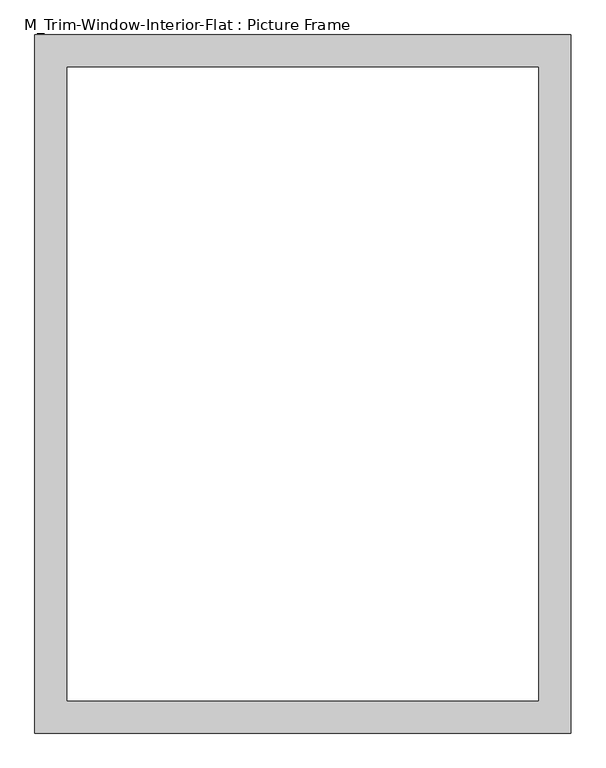
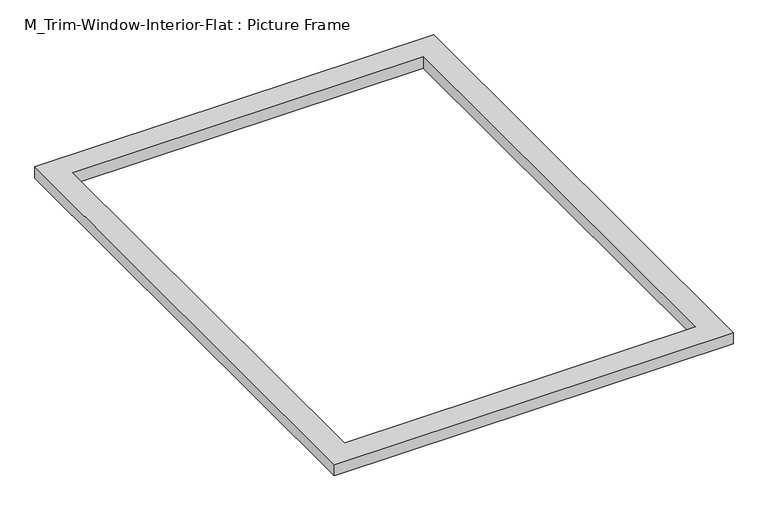
"""IFC4 building model written with IfcOpenShell, lengths in millimetres: proxy geometry, M_Trim-Window-Interior-Flat : Picture Frame."""

import ifcopenshell
import ifcopenshell.guid

model = None  # the IFC model being written
_history = None  # IfcOwnerHistory: only IFC2X3 demands one
_inside = {}  # id of a spatial element -> (the spatial element, [elements in it])
_under = {}  # id of a project, library or spatial element -> (it, [spatial elements below it])
_declared = {}  # id of a project -> (the project, [libraries it declares])
_typed = {}  # id of a type object -> (the type object, [elements of that type])
_made_of = {}  # id of a material, layer set ... -> (it, [elements and type objects made of it])


def new_model(schema):
    """Start an empty IFC model of exactly this schema.

    Asked for "IFC4X3", IfcOpenShell would pick the latest addendum, in which some entities
    have other attributes; the version numbers below select the first issue.
    IFC2X3 requires an IfcOwnerHistory on every rooted entity: one is made here for all.
    """
    global model, _history
    if schema == "IFC4X3":
        model = ifcopenshell.file(schema_version=(4, 3, 0, 0))
    else:
        model = ifcopenshell.file(schema=schema)
    _inside.clear()
    _under.clear()
    _declared.clear()
    _typed.clear()
    _made_of.clear()
    _history = None
    if model.schema == "IFC2X3":
        org = make("IfcOrganization", Name="unknown")
        user = make(
            "IfcPersonAndOrganization",
            ThePerson=make("IfcPerson", FamilyName="unknown"),
            TheOrganization=org,
        )
        app = make(
            "IfcApplication",
            ApplicationDeveloper=org,
            Version="unknown",
            ApplicationFullName="unknown",
            ApplicationIdentifier="unknown",
        )
        _history = make(
            "IfcOwnerHistory",
            OwningUser=user,
            OwningApplication=app,
            ChangeAction="ADDED",
            CreationDate=0,
        )
    return model


def make(cls, **values):
    """One entity of the class cls with the attributes given. An attribute that is None is left unset."""
    return model.create_entity(
        cls, **{name: value for name, value in values.items() if value is not None}
    )


def rooted(cls, **values):
    """An entity with a GlobalId (a new one), such as an element, a storey or a relation."""
    return make(cls, GlobalId=ifcopenshell.guid.new(), OwnerHistory=_history, **values)


def si_unit(unit_type, name, prefix=None):
    """IfcSIUnit, for example si_unit("LENGTHUNIT", "METRE", prefix="MILLI")."""
    return make("IfcSIUnit", UnitType=unit_type, Prefix=prefix, Name=name)


def assignment(units):
    """IfcUnitAssignment: the units of a project."""
    return None if units is None else make("IfcUnitAssignment", Units=units)


def point(xyz):
    """IfcCartesianPoint."""
    return None if xyz is None else make("IfcCartesianPoint", Coordinates=xyz)


def direction(xyz):
    """IfcDirection."""
    return None if xyz is None else make("IfcDirection", DirectionRatios=xyz)


def frame(location, z_axis=None, x_axis=None):
    """IfcAxis2Placement3D, a coordinate frame: its origin and axes. An axis left out is left unset."""
    return make(
        "IfcAxis2Placement3D",
        Location=point(location),
        Axis=direction(z_axis),
        RefDirection=direction(x_axis),
    )


def origin():
    """The frame at (0, 0, 0) with its axes left unset."""
    return frame((0.0, 0.0, 0.0))


def origin_with_axes():
    """The frame at (0, 0, 0) with the z axis (0, 0, 1) and the x axis (1, 0, 0) written out."""
    return frame((0.0, 0.0, 0.0), z_axis=(0.0, 0.0, 1.0), x_axis=(1.0, 0.0, 0.0))


def place(relative_to, where):
    """IfcLocalPlacement: puts the frame where relative to a parent placement (None: the world)."""
    return make(
        "IfcLocalPlacement", PlacementRelTo=relative_to, RelativePlacement=where
    )


def context(
    kind, dimensions, precision=None, world=None, true_north=None, identifier=None
):
    """IfcGeometricRepresentationContext, for example the 3D "Model" context."""
    return make(
        "IfcGeometricRepresentationContext",
        ContextIdentifier=identifier,
        ContextType=kind,
        CoordinateSpaceDimension=dimensions,
        Precision=precision,
        WorldCoordinateSystem=world,
        TrueNorth=true_north,
    )


def project(units=None, contexts=None):
    """IfcProject with its units and contexts."""
    return rooted(
        "IfcProject",
        Name="project",
        RepresentationContexts=contexts,
        UnitsInContext=assignment(units),
    )


def spatial(cls, under=None, at=None, **own):
    """A site, building, storey or space (cls), placed at a placement, below another one or the project."""
    s = rooted(cls, ObjectPlacement=at, **own)
    if under is not None:
        _under.setdefault(under.id(), (under, []))[1].append(s)
    return s


def polyline(points):
    """IfcPolyline through the points."""
    return make("IfcPolyline", Points=[point(p) for p in points])


def outline(outer, holes=None, kind="AREA"):
    """IfcArbitraryClosedProfileDef: a profile drawn as a closed curve; with holes, ...WithVoids."""
    if holes is None:
        return make("IfcArbitraryClosedProfileDef", ProfileType=kind, OuterCurve=outer)
    return make(
        "IfcArbitraryProfileDefWithVoids",
        ProfileType=kind,
        OuterCurve=outer,
        InnerCurves=holes,
    )


def extrude(swept, where, along, depth):
    """IfcExtrudedAreaSolid: the profile swept, set in the frame where, extruded along a direction by depth."""
    return make(
        "IfcExtrudedAreaSolid",
        SweptArea=swept,
        Position=where,
        ExtrudedDirection=direction(along),
        Depth=depth,
    )


def shape(context_of_items, identifier, shape_type, items):
    """IfcShapeRepresentation: the items that make up one representation, for example the "Body"."""
    return make(
        "IfcShapeRepresentation",
        ContextOfItems=context_of_items,
        RepresentationIdentifier=identifier,
        RepresentationType=shape_type,
        Items=items,
    )


def source(mapping_origin, context_of_items, identifier, shape_type, items):
    """IfcRepresentationMap: a shape defined once, which mapped items show again and again."""
    return make(
        "IfcRepresentationMap",
        MappingOrigin=mapping_origin,
        MappedRepresentation=shape(context_of_items, identifier, shape_type, items),
    )


def transform(
    local_origin,
    x_axis=None,
    y_axis=None,
    z_axis=None,
    scale=None,
    scale2=None,
    scale3=None,
    uniform=True,
):
    """IfcCartesianTransformationOperator3D, or its non-uniform kind. x_axis, y_axis, z_axis: its Axis1, 2, 3."""
    if uniform:
        return make(
            "IfcCartesianTransformationOperator3D",
            Axis1=direction(x_axis),
            Axis2=direction(y_axis),
            LocalOrigin=point(local_origin),
            Scale=scale,
            Axis3=direction(z_axis),
        )
    return make(
        "IfcCartesianTransformationOperator3DnonUniform",
        Axis1=direction(x_axis),
        Axis2=direction(y_axis),
        LocalOrigin=point(local_origin),
        Scale=scale,
        Axis3=direction(z_axis),
        Scale2=scale2,
        Scale3=scale3,
    )


def mapped(mapping_source, mapping_target):
    """IfcMappedItem: shows the shape of a source again, moved by a transform."""
    return make(
        "IfcMappedItem", MappingSource=mapping_source, MappingTarget=mapping_target
    )


def made_of(thing, what):
    """Note that an element or type object is made of a material, layer set ...; save() writes the relation."""
    if what is not None:
        _made_of.setdefault(what.id(), (what, []))[1].append(thing)
    return thing


def element(
    cls,
    number,
    at=None,
    inside=None,
    cuts=None,
    type_object=None,
    material=None,
    context=None,
    identifier="Body",
    shape_type=None,
    held_by="IfcProductDefinitionShape",
    body=None,
    shapes=None,
    **own,
):
    """One element of the class cls, such as IfcWall. Its Tag is "e" and its number.

    at: its placement. inside: the storey or other place that contains it. cuts: it is an
    opening in that element (IfcRelVoidsElement). A single representation is given by context,
    identifier, shape_type and body (its items); several are given by shapes. held_by: the class
    of the entity that holds the representations. save() writes the other relations.
    """
    e = rooted(cls, Tag="e%d" % number, ObjectPlacement=at, **own)
    if body is not None:
        shapes = [shape(context, identifier, shape_type, body)]
    if shapes is not None:
        e.Representation = make(held_by, Representations=shapes)
    if inside is not None:
        _inside.setdefault(inside.id(), (inside, []))[1].append(e)
    if cuts is not None:
        rooted(
            "IfcRelVoidsElement", RelatingBuildingElement=cuts, RelatedOpeningElement=e
        )
    if type_object is not None:
        _typed.setdefault(type_object.id(), (type_object, []))[1].append(e)
    return made_of(e, material)


def aggregate(whole, parts):
    """IfcRelAggregates: a whole, such as a stair, and the parts it consists of."""
    return rooted("IfcRelAggregates", RelatingObject=whole, RelatedObjects=parts)


def save(model, path):
    """Write the relations noted so far, then the file.

    IfcRelAggregates (storeys below a building ...), IfcRelContainedInSpatialStructure (elements
    in a storey), IfcRelDefinesByType, IfcRelAssociatesMaterial and IfcRelDeclares: one each for
    every whole, place, type object, material and project.
    """
    for whole, parts in _under.values():
        aggregate(whole, parts)
    for where, things in _inside.values():
        rooted(
            "IfcRelContainedInSpatialStructure",
            RelatedElements=things,
            RelatingStructure=where,
        )
    for kind, things in _typed.values():
        rooted("IfcRelDefinesByType", RelatedObjects=things, RelatingType=kind)
    for what, things in _made_of.values():
        rooted("IfcRelAssociatesMaterial", RelatedObjects=things, RelatingMaterial=what)
    for by, libraries in _declared.values():
        rooted("IfcRelDeclares", RelatingContext=by, RelatedDefinitions=libraries)
    model.write(path)


def m_trim_window_interior_flat_picture_frame_24fe8ef8(model_context):
    return source(origin(), model_context, "Body", "SweptSolid", [
        extrude(outline(polyline([(497.3, 47.3), (497.3, -1247.3), (-497.3, -1247.3), (-497.3, 47.3), (497.3, 47.3)]), holes=[polyline([(437.3, -12.7), (-437.3, -12.7), (-437.3, -1187.3), (437.3, -1187.3), (437.3, -12.7)])]), origin_with_axes(), (0.0, 0.0, 1.0), 30.0),
    ])


if __name__ == "__main__":
    model = new_model("IFC4")
    model_context = context("Model", 3, world=origin())
    ifc_project = project(units=[si_unit("LENGTHUNIT", "METRE", prefix="MILLI")], contexts=[model_context])
    site = spatial("IfcSite", under=ifc_project)
    building = spatial("IfcBuilding", under=site)
    placement = place(None, origin())
    m_trim_window_interior_flat_picture_frame_shape = m_trim_window_interior_flat_picture_frame_24fe8ef8(model_context)
    element("IfcBuildingElementProxy", 1, Name="M_Trim-Window-Interior-Flat : Picture Frame", ObjectType="M_Trim-Window-Interior-Flat : Picture Frame", at=placement, inside=building, context=model_context, shape_type="MappedRepresentation", body=[
        mapped(m_trim_window_interior_flat_picture_frame_shape, transform((0.0, 0.0, 0.0), x_axis=(1.0, 0.0, 0.0), y_axis=(0.0, 1.0, 0.0), z_axis=(0.0, 0.0, 1.0))),
    ])
    save(model, "model.ifc")

# Revit data of these elements
# Type "M_Trim-Window-Interior-Flat : Picture Frame"
#   Trim Thickness_Picture Frame = 30 mm
#   Trim Width = 60 mm
#   Trim Thickness_with Sill = 20 mm
#   Sill Thickness = 30 mm
#   Opening Width [instance default] = 600 mm
#   Opening Height [instance default] = 900 mm
#   Default Elevation = 1200 mm
#   Sill = no
#   Picture Frame = yes
#   Trim Material [instance default] = none
# Element 1 (IfcBuildingElementProxy, "M_Trim-Window-Interior-Flat : Picture Frame")
#   Opening Width = 900 mm
#   Opening Height = 1200 mm
#   Trim Material = Wood - Stained
#   Materials on its faces: "Wood - Stained"
# Materials
#   "Wood - Stained": class "Wood", colour RGB 173 132 96, transparency 0, Cost = 0
